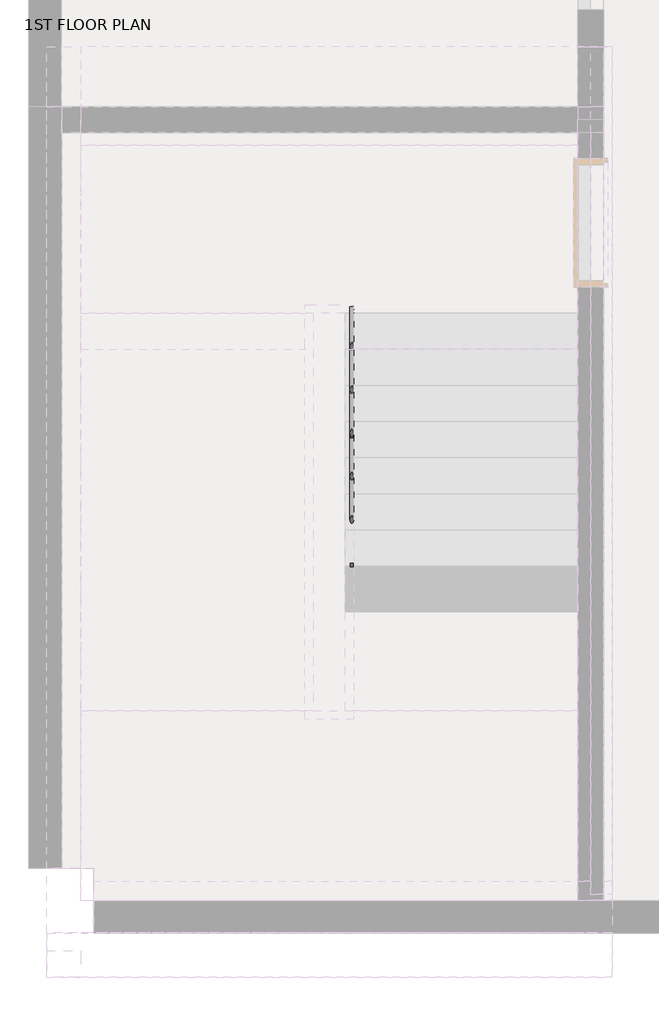
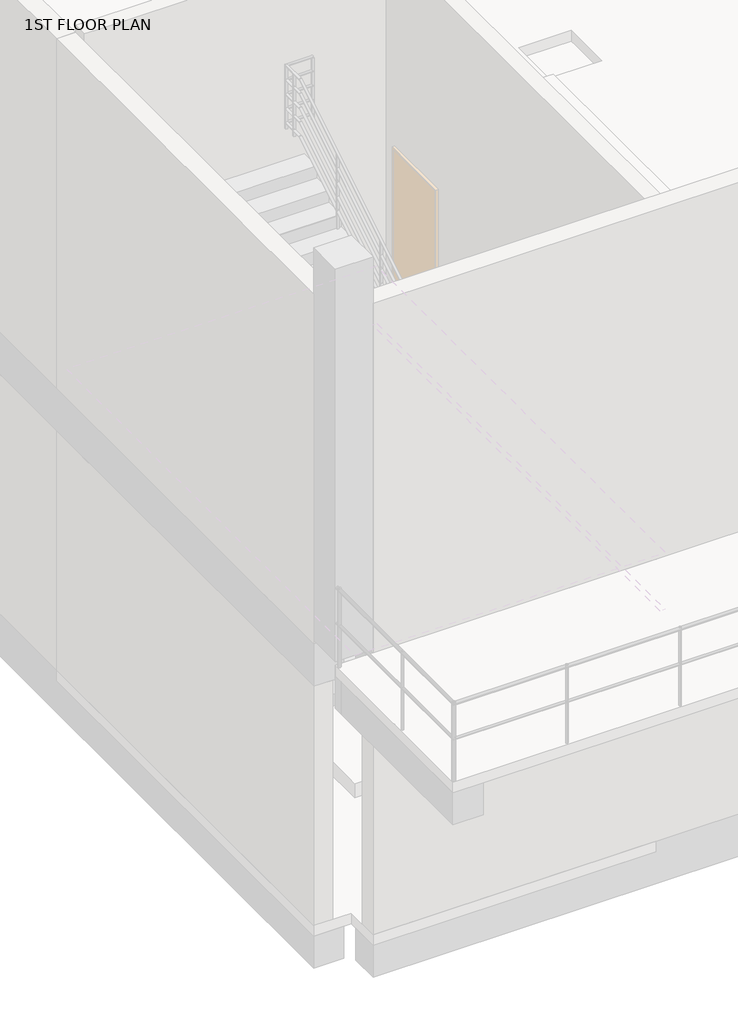
# One storey, part 7 of 9: 1 railing.
"""IFC4 building model written with IfcOpenShell, lengths in millimetres."""

from ifc_helpers import new_model, si_unit, frame, origin, place, context, project, spatial, polyline, circle_curve, ellipse_curve, outline, extrude, element, save
from ifc_brep_helpers import plane_surface, cylinder_surface, advanced_brep

model = new_model("IFC4")

# Units and contexts
model_context = context("Model", 3, world=origin())
ifc_project = project(units=[si_unit("LENGTHUNIT", "METRE", prefix="MILLI")], contexts=[model_context])

# Site, building, storey
site = spatial("IfcSite", under=ifc_project)
building = spatial("IfcBuilding", under=site)
storey = spatial("IfcBuildingStorey", under=building, Name="1ST FLOOR PLAN", Elevation=600.005241)

# Railing
placement = place(None, origin())
element("IfcRailing", 1, ObjectType="900mm 배관", at=placement, inside=storey, context=model_context, shape_type="SolidModel", body=[
    advanced_brep(
    [(2135.0, 25549.5208589, 1619.4537894), (2165.0, 25549.5208589, 1619.4537894), (2135.0, 22415.3944203, 3485.005241), (2165.0, 22415.3944203, 3485.005241), (2135.0, 22384.5208589, 3485.005241), (2165.0, 22354.5208589, 3485.005241), (1800.0, 22384.5208589, 3485.005241), (1800.0, 22354.5208589, 3485.005241)],
    [
        (0, 1, ellipse_curve(frame((2150.0, 25549.5208589, 1619.4537894), z_axis=(0.0, 1.0, 0.0), x_axis=(0.0, 0.0, -1.0)), 17.4562134, 15.0)),
        (1, 0, ellipse_curve(frame((2150.0, 25549.5208589, 1619.4537894), z_axis=(0.0, 1.0, 0.0), x_axis=(0.0, 0.0, -1.0)), 17.4562134, 15.0)),
        (0, 2),
        (2, 3, ellipse_curve(frame((2150.0, 22415.3944203, 3485.005241), z_axis=(0.0, 0.9641817474961643, -0.26524245096749255), x_axis=(0.0, -0.26524245096749166, -0.9641817474961646)), 15.5572329, 15.0)),
        (3, 1),
        (3, 2, ellipse_curve(frame((2150.0, 22415.3944203, 3485.005241), z_axis=(0.0, 0.9641817474961643, -0.26524245096749255), x_axis=(0.0, -0.26524245096749166, -0.9641817474961646)), 15.5572329, 15.0)),
        (2, 4),
        (4, 5, ellipse_curve(frame((2150.0, 22369.5208589, 3485.005241), z_axis=(0.7071067811865475, 0.7071067811865475, 0.0), x_axis=(-0.7071067811865474, 0.7071067811865476, 0.0)), 21.2132034, 15.0)),
        (5, 3),
        (5, 4, ellipse_curve(frame((2150.0, 22369.5208589, 3485.005241), z_axis=(0.7071067811865475, 0.7071067811865475, 0.0), x_axis=(-0.7071067811865474, 0.7071067811865476, 0.0)), 21.2132034, 15.0)),
        (6, 7, ellipse_curve(frame((1800.0, 22369.5208589, 3485.005241), z_axis=(-0.7071067811865476, 0.0, 0.7071067811865476), x_axis=(0.7071067811865474, 0.0, 0.7071067811865476)), 21.2132034, 15.0)),
        (7, 6, ellipse_curve(frame((1800.0, 22369.5208589, 3485.005241), z_axis=(-0.7071067811865476, 0.0, 0.7071067811865476), x_axis=(0.7071067811865474, 0.0, 0.7071067811865476)), 21.2132034, 15.0)),
        (4, 6),
        (7, 5),
    ],
    [
        plane_surface(frame((2150.0, 25549.5208589, 1636.9100029), z_axis=(0.0, 1.0, 0.0), x_axis=(0.0, 0.0, -1.0))),
        cylinder_surface(frame((2150.0, 25541.848601, 1624.0206096), z_axis=(0.0, 0.8592928844095147, -0.5114838597680054), x_axis=(1.0, 0.0, 0.0)), 15.0),
        cylinder_surface(frame((2150.0, 22419.5208589, 3485.005241), z_axis=(0.0, 1.0, 0.0), x_axis=(1.0, 0.0, 0.0)), 15.0),
        plane_surface(frame((1815.0, 22369.5208589, 3500.005241), z_axis=(-0.7071067811865476, 0.0, 0.7071067811865476), x_axis=(0.7071067811865476, 0.0, 0.7071067811865476))),
        cylinder_surface(frame((2150.0, 22369.5208589, 3485.005241), z_axis=(1.0, 0.0, 0.0), x_axis=(0.0, -1.0, 0.0)), 15.0),
    ],
    [
        (0, [[1, 2]]),
        (1, [[-1, 3, 4, 5]]),
        (1, [[-2, -5, 6, -3]]),
        (2, [[-4, 7, 8, 9]]),
        (2, [[-6, -9, 10, -7]]),
        (3, [[11, 12]]),
        (4, [[-8, 13, -12, 14]]),
        (4, [[-10, -14, -11, -13]]),
    ],
),
    advanced_brep(
    [(1800.0, 22384.5208589, 3485.005241), (1800.0, 22354.5208589, 3485.005241), (1800.0, 22384.5208589, 3610.9261474), (1800.0, 22354.5208589, 3627.9814314)],
    [
        (0, 1, ellipse_curve(frame((1800.0, 22369.5208589, 3485.005241), z_axis=(0.7071067811865476, 0.0, -0.7071067811865476), x_axis=(-0.7071067811865476, 0.0, -0.7071067811865474)), 21.2132034, 15.0)),
        (1, 0, ellipse_curve(frame((1800.0, 22369.5208589, 3485.005241), z_axis=(0.7071067811865476, 0.0, -0.7071067811865476), x_axis=(-0.7071067811865476, 0.0, -0.7071067811865474)), 21.2132034, 15.0)),
        (2, 3, ellipse_curve(frame((1800.0, 22369.5208589, 3619.4537894), z_axis=(0.0, 0.4942247162131791, 0.8693341876884877), x_axis=(0.0, 0.8693341876884879, -0.49422471621317876)), 17.2545843, 15.0)),
        (3, 2, ellipse_curve(frame((1800.0, 22369.5208589, 3619.4537894), z_axis=(0.0, 0.4942247162131791, 0.8693341876884877), x_axis=(0.0, 0.8693341876884879, -0.49422471621317876)), 17.2545843, 15.0)),
        (0, 2),
        (3, 1),
    ],
    [
        plane_surface(frame((1800.0, 22369.5208589, 3485.005241), z_axis=(0.7071067811865476, 0.0, -0.7071067811865476), x_axis=(0.7071067811865476, 0.0, 0.7071067811865476))),
        plane_surface(frame((1800.0, 22369.5208589, 3619.4537894), z_axis=(0.0, 0.4942247162131791, 0.8693341876884877), x_axis=(1.0, 0.0, 0.0))),
        cylinder_surface(frame((1800.0, 22369.5208589, 3485.005241), z_axis=(0.0, 0.0, -1.0), x_axis=(0.0, -1.0, 0.0)), 15.0),
    ],
    [
        (0, [[1, 2]]),
        (1, [[3, 4]]),
        (2, [[-1, 5, -4, 6]]),
        (2, [[-2, -6, -3, -5]]),
    ],
),
    advanced_brep(
    [(1815.0, 22369.5208589, 3619.4537894), (1785.0, 22369.5208589, 3619.4537894), (1815.0, 25503.6472975, 5485.005241), (1785.0, 25503.6472975, 5485.005241), (1815.0, 25534.5208589, 5485.005241), (1785.0, 25564.5208589, 5485.005241), (2150.0, 25534.5208589, 5485.005241), (2150.0, 25564.5208589, 5485.005241)],
    [
        (0, 1, ellipse_curve(frame((1800.0, 22369.5208589, 3619.4537894), z_axis=(0.0, -0.4942247162131791, -0.8693341876884877), x_axis=(0.0, -0.8693341876884876, 0.49422471621317926)), 17.2545843, 15.0)),
        (1, 0, ellipse_curve(frame((1800.0, 22369.5208589, 3619.4537894), z_axis=(0.0, -0.4942247162131791, -0.8693341876884877), x_axis=(0.0, -0.8693341876884876, 0.49422471621317926)), 17.2545843, 15.0)),
        (0, 2),
        (2, 3, ellipse_curve(frame((1800.0, 25503.6472975, 5485.005241), z_axis=(0.0, -0.9641817474961643, -0.26524245096749255), x_axis=(0.0, 0.26524245096749166, -0.9641817474961646)), 15.5572329, 15.0)),
        (3, 1),
        (3, 2, ellipse_curve(frame((1800.0, 25503.6472975, 5485.005241), z_axis=(0.0, -0.9641817474961643, -0.26524245096749255), x_axis=(0.0, 0.26524245096749166, -0.9641817474961646)), 15.5572329, 15.0)),
        (2, 4),
        (4, 5, ellipse_curve(frame((1800.0, 25549.5208589, 5485.005241), z_axis=(-0.7071067811865475, -0.7071067811865475, 0.0), x_axis=(0.7071067811865474, -0.7071067811865476, 0.0)), 21.2132034, 15.0)),
        (5, 3),
        (5, 4, ellipse_curve(frame((1800.0, 25549.5208589, 5485.005241), z_axis=(-0.7071067811865475, -0.7071067811865475, 0.0), x_axis=(0.7071067811865474, -0.7071067811865476, 0.0)), 21.2132034, 15.0)),
        (6, 7, circle_curve(frame((2150.0, 25549.5208589, 5485.005241), z_axis=(1.0, 0.0, 0.0), x_axis=(0.0, 1.0, 0.0)), 15.0)),
        (7, 6, circle_curve(frame((2150.0, 25549.5208589, 5485.005241), z_axis=(1.0, 0.0, 0.0), x_axis=(0.0, 1.0, 0.0)), 15.0)),
        (4, 6),
        (7, 5),
    ],
    [
        plane_surface(frame((1800.0, 22354.5208589, 3627.9814314), z_axis=(0.0, -0.4942247162131791, -0.8693341876884877), x_axis=(1.0, 0.0, 0.0))),
        cylinder_surface(frame((1800.0, 22362.1931168, 3615.0920382), z_axis=(0.0, -0.8592928844095147, -0.5114838597680054), x_axis=(-1.0, 0.0, 0.0)), 15.0),
        cylinder_surface(frame((1800.0, 25499.5208589, 5485.005241), z_axis=(0.0, -1.0, 0.0), x_axis=(-1.0, 0.0, 0.0)), 15.0),
        plane_surface(frame((2150.0, 25549.5208589, 5500.005241), z_axis=(1.0, 0.0, 0.0), x_axis=(0.0, 1.0, 0.0))),
        cylinder_surface(frame((1800.0, 25549.5208589, 5485.005241), z_axis=(-1.0, 0.0, 0.0), x_axis=(0.0, 1.0, 0.0)), 15.0),
    ],
    [
        (0, [[1, 2]]),
        (1, [[-1, 3, 4, 5]]),
        (1, [[-2, -5, 6, -3]]),
        (2, [[-4, 7, 8, 9]]),
        (2, [[-6, -9, 10, -7]]),
        (3, [[11, 12]]),
        (4, [[-8, 13, -12, 14]]),
        (4, [[-10, -14, -11, -13]]),
    ],
),
    advanced_brep(
    [(2165.0, 25549.5208589, 1419.4537894), (2135.0, 25549.5208589, 1419.4537894), (2165.0, 22415.3944203, 3285.005241), (2135.0, 22415.3944203, 3285.005241), (2165.0, 22384.5208589, 3285.005241), (2135.0, 22384.5208589, 3285.005241)],
    [
        (0, 1, ellipse_curve(frame((2150.0, 25549.5208589, 1419.4537894), z_axis=(0.0, 1.0, 0.0), x_axis=(0.0, 0.0, -1.0)), 17.4562134, 15.0)),
        (1, 0, ellipse_curve(frame((2150.0, 25549.5208589, 1419.4537894), z_axis=(0.0, 1.0, 0.0), x_axis=(0.0, 0.0, -1.0)), 17.4562134, 15.0)),
        (0, 2),
        (2, 3, ellipse_curve(frame((2150.0, 22415.3944203, 3285.005241), z_axis=(0.0, 0.9641817474961643, -0.26524245096749255), x_axis=(0.0, -0.26524245096749166, -0.9641817474961646)), 15.5572329, 15.0)),
        (3, 1),
        (3, 2, ellipse_curve(frame((2150.0, 22415.3944203, 3285.005241), z_axis=(0.0, 0.9641817474961643, -0.26524245096749255), x_axis=(0.0, -0.26524245096749166, -0.9641817474961646)), 15.5572329, 15.0)),
        (4, 5, circle_curve(frame((2150.0, 22384.5208589, 3285.005241), z_axis=(0.0, -1.0, 0.0), x_axis=(-1.0, 0.0, 0.0)), 15.0)),
        (5, 4, circle_curve(frame((2150.0, 22384.5208589, 3285.005241), z_axis=(0.0, -1.0, 0.0), x_axis=(-1.0, 0.0, 0.0)), 15.0)),
        (2, 4),
        (5, 3),
    ],
    [
        plane_surface(frame((2150.0, 25549.5208589, 1436.9100029), z_axis=(0.0, 1.0, 0.0), x_axis=(0.0, 0.0, -1.0))),
        cylinder_surface(frame((2150.0, 25541.848601, 1424.0206096), z_axis=(0.0, 0.8592928844095147, -0.5114838597680054), x_axis=(-1.0, 0.0, 0.0)), 15.0),
        plane_surface(frame((2150.0, 22384.5208589, 3300.005241), z_axis=(0.0, -1.0, 0.0), x_axis=(0.0, 0.0, -1.0))),
        cylinder_surface(frame((2150.0, 22419.5208589, 3285.005241), z_axis=(0.0, 1.0, 0.0), x_axis=(-1.0, 0.0, 0.0)), 15.0),
    ],
    [
        (0, [[1, 2]]),
        (1, [[-1, 3, 4, 5]]),
        (1, [[-2, -5, 6, -3]]),
        (2, [[7, 8]]),
        (3, [[-4, 9, -8, 10]]),
        (3, [[-6, -10, -7, -9]]),
    ],
),
    advanced_brep(
    [(2165.0, 22354.5208589, 3285.005241), (2165.0, 22384.5208589, 3285.005241), (1815.0, 22354.5208589, 3285.005241), (1815.0, 22384.5208589, 3285.005241)],
    [
        (0, 1, circle_curve(frame((2165.0, 22369.5208589, 3285.005241), z_axis=(1.0, 0.0, 0.0), x_axis=(0.0, 1.0, 0.0)), 15.0)),
        (1, 0, circle_curve(frame((2165.0, 22369.5208589, 3285.005241), z_axis=(1.0, 0.0, 0.0), x_axis=(0.0, 1.0, 0.0)), 15.0)),
        (2, 3, circle_curve(frame((1815.0, 22369.5208589, 3285.005241), z_axis=(-1.0, 0.0, 0.0), x_axis=(0.0, 1.0, 0.0)), 15.0)),
        (3, 2, circle_curve(frame((1815.0, 22369.5208589, 3285.005241), z_axis=(-1.0, 0.0, 0.0), x_axis=(0.0, 1.0, 0.0)), 15.0)),
        (0, 2),
        (3, 1),
    ],
    [
        plane_surface(frame((2165.0, 22369.5208589, 3300.005241), z_axis=(1.0, 0.0, 0.0), x_axis=(0.0, -1.0, 0.0))),
        plane_surface(frame((1815.0, 22369.5208589, 3300.005241), z_axis=(-1.0, 0.0, 0.0), x_axis=(0.0, -1.0, 0.0))),
        cylinder_surface(frame((2165.0, 22369.5208589, 3285.005241), z_axis=(1.0, 0.0, 0.0), x_axis=(0.0, 1.0, 0.0)), 15.0),
    ],
    [
        (0, [[1, 2]]),
        (1, [[3, 4]]),
        (2, [[-1, 5, -4, 6]]),
        (2, [[-2, -6, -3, -5]]),
    ],
),
    advanced_brep(
    [(1785.0, 22354.5208589, 3410.525218), (1815.0, 22354.5208589, 3410.525218), (1785.0, 25503.6472975, 5285.005241), (1815.0, 25503.6472975, 5285.005241), (1785.0, 25534.5208589, 5285.005241), (1815.0, 25534.5208589, 5285.005241)],
    [
        (0, 1, ellipse_curve(frame((1800.0, 22354.5208589, 3410.525218), z_axis=(0.0, -1.0, 0.0), x_axis=(0.0, 0.0, -1.0)), 17.4562134, 15.0)),
        (1, 0, ellipse_curve(frame((1800.0, 22354.5208589, 3410.525218), z_axis=(0.0, -1.0, 0.0), x_axis=(0.0, 0.0, -1.0)), 17.4562134, 15.0)),
        (0, 2),
        (2, 3, ellipse_curve(frame((1800.0, 25503.6472975, 5285.005241), z_axis=(0.0, -0.9641817474961643, -0.26524245096749255), x_axis=(0.0, 0.26524245096749166, -0.9641817474961646)), 15.5572329, 15.0)),
        (3, 1),
        (3, 2, ellipse_curve(frame((1800.0, 25503.6472975, 5285.005241), z_axis=(0.0, -0.9641817474961643, -0.26524245096749255), x_axis=(0.0, 0.26524245096749166, -0.9641817474961646)), 15.5572329, 15.0)),
        (4, 5, circle_curve(frame((1800.0, 25534.5208589, 5285.005241), z_axis=(0.0, 1.0, 0.0), x_axis=(1.0, 0.0, 0.0)), 15.0)),
        (5, 4, circle_curve(frame((1800.0, 25534.5208589, 5285.005241), z_axis=(0.0, 1.0, 0.0), x_axis=(1.0, 0.0, 0.0)), 15.0)),
        (2, 4),
        (5, 3),
    ],
    [
        plane_surface(frame((1800.0, 22354.5208589, 3427.9814314), z_axis=(0.0, -1.0, 0.0), x_axis=(0.0, 0.0, 1.0))),
        cylinder_surface(frame((1800.0, 22362.1931168, 3415.0920382), z_axis=(0.0, -0.8592928844095147, -0.5114838597680054), x_axis=(1.0, 0.0, 0.0)), 15.0),
        plane_surface(frame((1800.0, 25534.5208589, 5300.005241), z_axis=(0.0, 1.0, 0.0), x_axis=(0.0, 0.0, 1.0))),
        cylinder_surface(frame((1800.0, 25499.5208589, 5285.005241), z_axis=(0.0, -1.0, 0.0), x_axis=(1.0, 0.0, 0.0)), 15.0),
    ],
    [
        (0, [[1, 2]]),
        (1, [[-1, 3, 4, 5]]),
        (1, [[-2, -5, 6, -3]]),
        (2, [[7, 8]]),
        (3, [[-4, 9, -8, 10]]),
        (3, [[-6, -10, -7, -9]]),
    ],
),
    advanced_brep(
    [(1785.0, 25564.5208589, 5285.005241), (1785.0, 25534.5208589, 5285.005241), (2150.0, 25564.5208589, 5285.005241), (2150.0, 25534.5208589, 5285.005241)],
    [
        (0, 1, circle_curve(frame((1785.0, 25549.5208589, 5285.005241), z_axis=(-1.0, 0.0, 0.0), x_axis=(0.0, -1.0, 0.0)), 15.0)),
        (1, 0, circle_curve(frame((1785.0, 25549.5208589, 5285.005241), z_axis=(-1.0, 0.0, 0.0), x_axis=(0.0, -1.0, 0.0)), 15.0)),
        (2, 3, circle_curve(frame((2150.0, 25549.5208589, 5285.005241), z_axis=(1.0, 0.0, 0.0), x_axis=(0.0, -1.0, 0.0)), 15.0)),
        (3, 2, circle_curve(frame((2150.0, 25549.5208589, 5285.005241), z_axis=(1.0, 0.0, 0.0), x_axis=(0.0, -1.0, 0.0)), 15.0)),
        (0, 2),
        (3, 1),
    ],
    [
        plane_surface(frame((1785.0, 25549.5208589, 5300.005241), z_axis=(-1.0, 0.0, 0.0), x_axis=(0.0, 1.0, 0.0))),
        plane_surface(frame((2150.0, 25549.5208589, 5300.005241), z_axis=(1.0, 0.0, 0.0), x_axis=(0.0, 1.0, 0.0))),
        cylinder_surface(frame((1785.0, 25549.5208589, 5285.005241), z_axis=(-1.0, 0.0, 0.0), x_axis=(0.0, -1.0, 0.0)), 15.0),
    ],
    [
        (0, [[1, 2]]),
        (1, [[3, 4]]),
        (2, [[-1, 5, -4, 6]]),
        (2, [[-2, -6, -3, -5]]),
    ],
),
    advanced_brep(
    [(2165.0, 25549.5208589, 1219.4537894), (2135.0, 25549.5208589, 1219.4537894), (2165.0, 22415.3944203, 3085.005241), (2135.0, 22415.3944203, 3085.005241), (2165.0, 22384.5208589, 3085.005241), (2135.0, 22384.5208589, 3085.005241)],
    [
        (0, 1, ellipse_curve(frame((2150.0, 25549.5208589, 1219.4537894), z_axis=(0.0, 1.0, 0.0), x_axis=(0.0, 0.0, -1.0)), 17.4562134, 15.0)),
        (1, 0, ellipse_curve(frame((2150.0, 25549.5208589, 1219.4537894), z_axis=(0.0, 1.0, 0.0), x_axis=(0.0, 0.0, -1.0)), 17.4562134, 15.0)),
        (0, 2),
        (2, 3, ellipse_curve(frame((2150.0, 22415.3944203, 3085.005241), z_axis=(0.0, 0.9641817474961643, -0.26524245096749255), x_axis=(0.0, -0.26524245096749166, -0.9641817474961646)), 15.5572329, 15.0)),
        (3, 1),
        (3, 2, ellipse_curve(frame((2150.0, 22415.3944203, 3085.005241), z_axis=(0.0, 0.9641817474961643, -0.26524245096749255), x_axis=(0.0, -0.26524245096749166, -0.9641817474961646)), 15.5572329, 15.0)),
        (4, 5, circle_curve(frame((2150.0, 22384.5208589, 3085.005241), z_axis=(0.0, -1.0, 0.0), x_axis=(-1.0, 0.0, 0.0)), 15.0)),
        (5, 4, circle_curve(frame((2150.0, 22384.5208589, 3085.005241), z_axis=(0.0, -1.0, 0.0), x_axis=(-1.0, 0.0, 0.0)), 15.0)),
        (2, 4),
        (5, 3),
    ],
    [
        plane_surface(frame((2150.0, 25549.5208589, 1236.9100029), z_axis=(0.0, 1.0, 0.0), x_axis=(0.0, 0.0, -1.0))),
        cylinder_surface(frame((2150.0, 25541.848601, 1224.0206096), z_axis=(0.0, 0.8592928844095147, -0.5114838597680054), x_axis=(-1.0, 0.0, 0.0)), 15.0),
        plane_surface(frame((2150.0, 22384.5208589, 3100.005241), z_axis=(0.0, -1.0, 0.0), x_axis=(0.0, 0.0, -1.0))),
        cylinder_surface(frame((2150.0, 22419.5208589, 3085.005241), z_axis=(0.0, 1.0, 0.0), x_axis=(-1.0, 0.0, 0.0)), 15.0),
    ],
    [
        (0, [[1, 2]]),
        (1, [[-1, 3, 4, 5]]),
        (1, [[-2, -5, 6, -3]]),
        (2, [[7, 8]]),
        (3, [[-4, 9, -8, 10]]),
        (3, [[-6, -10, -7, -9]]),
    ],
),
    advanced_brep(
    [(2165.0, 22354.5208589, 3085.005241), (2165.0, 22384.5208589, 3085.005241), (1815.0, 22354.5208589, 3085.005241), (1815.0, 22384.5208589, 3085.005241)],
    [
        (0, 1, circle_curve(frame((2165.0, 22369.5208589, 3085.005241), z_axis=(1.0, 0.0, 0.0), x_axis=(0.0, 1.0, 0.0)), 15.0)),
        (1, 0, circle_curve(frame((2165.0, 22369.5208589, 3085.005241), z_axis=(1.0, 0.0, 0.0), x_axis=(0.0, 1.0, 0.0)), 15.0)),
        (2, 3, circle_curve(frame((1815.0, 22369.5208589, 3085.005241), z_axis=(-1.0, 0.0, 0.0), x_axis=(0.0, 1.0, 0.0)), 15.0)),
        (3, 2, circle_curve(frame((1815.0, 22369.5208589, 3085.005241), z_axis=(-1.0, 0.0, 0.0), x_axis=(0.0, 1.0, 0.0)), 15.0)),
        (0, 2),
        (3, 1),
    ],
    [
        plane_surface(frame((2165.0, 22369.5208589, 3100.005241), z_axis=(1.0, 0.0, 0.0), x_axis=(0.0, -1.0, 0.0))),
        plane_surface(frame((1815.0, 22369.5208589, 3100.005241), z_axis=(-1.0, 0.0, 0.0), x_axis=(0.0, -1.0, 0.0))),
        cylinder_surface(frame((2165.0, 22369.5208589, 3085.005241), z_axis=(1.0, 0.0, 0.0), x_axis=(0.0, 1.0, 0.0)), 15.0),
    ],
    [
        (0, [[1, 2]]),
        (1, [[3, 4]]),
        (2, [[-1, 5, -4, 6]]),
        (2, [[-2, -6, -3, -5]]),
    ],
),
    advanced_brep(
    [(1785.0, 22354.5208589, 3210.525218), (1815.0, 22354.5208589, 3210.525218), (1785.0, 25503.6472975, 5085.005241), (1815.0, 25503.6472975, 5085.005241), (1785.0, 25534.5208589, 5085.005241), (1815.0, 25534.5208589, 5085.005241)],
    [
        (0, 1, ellipse_curve(frame((1800.0, 22354.5208589, 3210.525218), z_axis=(0.0, -1.0, 0.0), x_axis=(0.0, 0.0, -1.0)), 17.4562134, 15.0)),
        (1, 0, ellipse_curve(frame((1800.0, 22354.5208589, 3210.525218), z_axis=(0.0, -1.0, 0.0), x_axis=(0.0, 0.0, -1.0)), 17.4562134, 15.0)),
        (0, 2),
        (2, 3, ellipse_curve(frame((1800.0, 25503.6472975, 5085.005241), z_axis=(0.0, -0.9641817474961643, -0.26524245096749255), x_axis=(0.0, 0.26524245096749166, -0.9641817474961646)), 15.5572329, 15.0)),
        (3, 1),
        (3, 2, ellipse_curve(frame((1800.0, 25503.6472975, 5085.005241), z_axis=(0.0, -0.9641817474961643, -0.26524245096749255), x_axis=(0.0, 0.26524245096749166, -0.9641817474961646)), 15.5572329, 15.0)),
        (4, 5, circle_curve(frame((1800.0, 25534.5208589, 5085.005241), z_axis=(0.0, 1.0, 0.0), x_axis=(1.0, 0.0, 0.0)), 15.0)),
        (5, 4, circle_curve(frame((1800.0, 25534.5208589, 5085.005241), z_axis=(0.0, 1.0, 0.0), x_axis=(1.0, 0.0, 0.0)), 15.0)),
        (2, 4),
        (5, 3),
    ],
    [
        plane_surface(frame((1800.0, 22354.5208589, 3227.9814314), z_axis=(0.0, -1.0, 0.0), x_axis=(0.0, 0.0, 1.0))),
        cylinder_surface(frame((1800.0, 22362.1931168, 3215.0920382), z_axis=(0.0, -0.8592928844095147, -0.5114838597680054), x_axis=(1.0, 0.0, 0.0)), 15.0),
        plane_surface(frame((1800.0, 25534.5208589, 5100.005241), z_axis=(0.0, 1.0, 0.0), x_axis=(0.0, 0.0, 1.0))),
        cylinder_surface(frame((1800.0, 25499.5208589, 5085.005241), z_axis=(0.0, -1.0, 0.0), x_axis=(1.0, 0.0, 0.0)), 15.0),
    ],
    [
        (0, [[1, 2]]),
        (1, [[-1, 3, 4, 5]]),
        (1, [[-2, -5, 6, -3]]),
        (2, [[7, 8]]),
        (3, [[-4, 9, -8, 10]]),
        (3, [[-6, -10, -7, -9]]),
    ],
),
    advanced_brep(
    [(1785.0, 25564.5208589, 5085.005241), (1785.0, 25534.5208589, 5085.005241), (2150.0, 25564.5208589, 5085.005241), (2150.0, 25534.5208589, 5085.005241)],
    [
        (0, 1, circle_curve(frame((1785.0, 25549.5208589, 5085.005241), z_axis=(-1.0, 0.0, 0.0), x_axis=(0.0, -1.0, 0.0)), 15.0)),
        (1, 0, circle_curve(frame((1785.0, 25549.5208589, 5085.005241), z_axis=(-1.0, 0.0, 0.0), x_axis=(0.0, -1.0, 0.0)), 15.0)),
        (2, 3, circle_curve(frame((2150.0, 25549.5208589, 5085.005241), z_axis=(1.0, 0.0, 0.0), x_axis=(0.0, -1.0, 0.0)), 15.0)),
        (3, 2, circle_curve(frame((2150.0, 25549.5208589, 5085.005241), z_axis=(1.0, 0.0, 0.0), x_axis=(0.0, -1.0, 0.0)), 15.0)),
        (0, 2),
        (3, 1),
    ],
    [
        plane_surface(frame((1785.0, 25549.5208589, 5100.005241), z_axis=(-1.0, 0.0, 0.0), x_axis=(0.0, 1.0, 0.0))),
        plane_surface(frame((2150.0, 25549.5208589, 5100.005241), z_axis=(1.0, 0.0, 0.0), x_axis=(0.0, 1.0, 0.0))),
        cylinder_surface(frame((1785.0, 25549.5208589, 5085.005241), z_axis=(-1.0, 0.0, 0.0), x_axis=(0.0, -1.0, 0.0)), 15.0),
    ],
    [
        (0, [[1, 2]]),
        (1, [[3, 4]]),
        (2, [[-1, 5, -4, 6]]),
        (2, [[-2, -6, -3, -5]]),
    ],
),
    advanced_brep(
    [(2165.0, 25549.5208589, 1019.4537894), (2135.0, 25549.5208589, 1019.4537894), (2165.0, 22415.3944203, 2885.005241), (2135.0, 22415.3944203, 2885.005241), (2165.0, 22384.5208589, 2885.005241), (2135.0, 22384.5208589, 2885.005241)],
    [
        (0, 1, ellipse_curve(frame((2150.0, 25549.5208589, 1019.4537894), z_axis=(0.0, 1.0, 0.0), x_axis=(0.0, 0.0, -1.0)), 17.4562134, 15.0)),
        (1, 0, ellipse_curve(frame((2150.0, 25549.5208589, 1019.4537894), z_axis=(0.0, 1.0, 0.0), x_axis=(0.0, 0.0, -1.0)), 17.4562134, 15.0)),
        (0, 2),
        (2, 3, ellipse_curve(frame((2150.0, 22415.3944203, 2885.005241), z_axis=(0.0, 0.9641817474961643, -0.26524245096749255), x_axis=(0.0, -0.26524245096749166, -0.9641817474961646)), 15.5572329, 15.0)),
        (3, 1),
        (3, 2, ellipse_curve(frame((2150.0, 22415.3944203, 2885.005241), z_axis=(0.0, 0.9641817474961643, -0.26524245096749255), x_axis=(0.0, -0.26524245096749166, -0.9641817474961646)), 15.5572329, 15.0)),
        (4, 5, circle_curve(frame((2150.0, 22384.5208589, 2885.005241), z_axis=(0.0, -1.0, 0.0), x_axis=(-1.0, 0.0, 0.0)), 15.0)),
        (5, 4, circle_curve(frame((2150.0, 22384.5208589, 2885.005241), z_axis=(0.0, -1.0, 0.0), x_axis=(-1.0, 0.0, 0.0)), 15.0)),
        (2, 4),
        (5, 3),
    ],
    [
        plane_surface(frame((2150.0, 25549.5208589, 1036.9100029), z_axis=(0.0, 1.0, 0.0), x_axis=(0.0, 0.0, -1.0))),
        cylinder_surface(frame((2150.0, 25541.848601, 1024.0206096), z_axis=(0.0, 0.8592928844095147, -0.5114838597680054), x_axis=(-1.0, 0.0, 0.0)), 15.0),
        plane_surface(frame((2150.0, 22384.5208589, 2900.005241), z_axis=(0.0, -1.0, 0.0), x_axis=(0.0, 0.0, -1.0))),
        cylinder_surface(frame((2150.0, 22419.5208589, 2885.005241), z_axis=(0.0, 1.0, 0.0), x_axis=(-1.0, 0.0, 0.0)), 15.0),
    ],
    [
        (0, [[1, 2]]),
        (1, [[-1, 3, 4, 5]]),
        (1, [[-2, -5, 6, -3]]),
        (2, [[7, 8]]),
        (3, [[-4, 9, -8, 10]]),
        (3, [[-6, -10, -7, -9]]),
    ],
),
    advanced_brep(
    [(2165.0, 22354.5208589, 2885.005241), (2165.0, 22384.5208589, 2885.005241), (1815.0, 22354.5208589, 2885.005241), (1815.0, 22384.5208589, 2885.005241)],
    [
        (0, 1, circle_curve(frame((2165.0, 22369.5208589, 2885.005241), z_axis=(1.0, 0.0, 0.0), x_axis=(0.0, 1.0, 0.0)), 15.0)),
        (1, 0, circle_curve(frame((2165.0, 22369.5208589, 2885.005241), z_axis=(1.0, 0.0, 0.0), x_axis=(0.0, 1.0, 0.0)), 15.0)),
        (2, 3, circle_curve(frame((1815.0, 22369.5208589, 2885.005241), z_axis=(-1.0, 0.0, 0.0), x_axis=(0.0, 1.0, 0.0)), 15.0)),
        (3, 2, circle_curve(frame((1815.0, 22369.5208589, 2885.005241), z_axis=(-1.0, 0.0, 0.0), x_axis=(0.0, 1.0, 0.0)), 15.0)),
        (0, 2),
        (3, 1),
    ],
    [
        plane_surface(frame((2165.0, 22369.5208589, 2900.005241), z_axis=(1.0, 0.0, 0.0), x_axis=(0.0, -1.0, 0.0))),
        plane_surface(frame((1815.0, 22369.5208589, 2900.005241), z_axis=(-1.0, 0.0, 0.0), x_axis=(0.0, -1.0, 0.0))),
        cylinder_surface(frame((2165.0, 22369.5208589, 2885.005241), z_axis=(1.0, 0.0, 0.0), x_axis=(0.0, 1.0, 0.0)), 15.0),
    ],
    [
        (0, [[1, 2]]),
        (1, [[3, 4]]),
        (2, [[-1, 5, -4, 6]]),
        (2, [[-2, -6, -3, -5]]),
    ],
),
    advanced_brep(
    [(1785.0, 22354.5208589, 3010.525218), (1815.0, 22354.5208589, 3010.525218), (1785.0, 25503.6472975, 4885.005241), (1815.0, 25503.6472975, 4885.005241), (1785.0, 25534.5208589, 4885.005241), (1815.0, 25534.5208589, 4885.005241)],
    [
        (0, 1, ellipse_curve(frame((1800.0, 22354.5208589, 3010.525218), z_axis=(0.0, -1.0, 0.0), x_axis=(0.0, 0.0, -1.0)), 17.4562134, 15.0)),
        (1, 0, ellipse_curve(frame((1800.0, 22354.5208589, 3010.525218), z_axis=(0.0, -1.0, 0.0), x_axis=(0.0, 0.0, -1.0)), 17.4562134, 15.0)),
        (0, 2),
        (2, 3, ellipse_curve(frame((1800.0, 25503.6472975, 4885.005241), z_axis=(0.0, -0.9641817474961643, -0.26524245096749255), x_axis=(0.0, 0.26524245096749166, -0.9641817474961646)), 15.5572329, 15.0)),
        (3, 1),
        (3, 2, ellipse_curve(frame((1800.0, 25503.6472975, 4885.005241), z_axis=(0.0, -0.9641817474961643, -0.26524245096749255), x_axis=(0.0, 0.26524245096749166, -0.9641817474961646)), 15.5572329, 15.0)),
        (4, 5, circle_curve(frame((1800.0, 25534.5208589, 4885.005241), z_axis=(0.0, 1.0, 0.0), x_axis=(1.0, 0.0, 0.0)), 15.0)),
        (5, 4, circle_curve(frame((1800.0, 25534.5208589, 4885.005241), z_axis=(0.0, 1.0, 0.0), x_axis=(1.0, 0.0, 0.0)), 15.0)),
        (2, 4),
        (5, 3),
    ],
    [
        plane_surface(frame((1800.0, 22354.5208589, 3027.9814314), z_axis=(0.0, -1.0, 0.0), x_axis=(0.0, 0.0, 1.0))),
        cylinder_surface(frame((1800.0, 22362.1931168, 3015.0920382), z_axis=(0.0, -0.8592928844095147, -0.5114838597680054), x_axis=(1.0, 0.0, 0.0)), 15.0),
        plane_surface(frame((1800.0, 25534.5208589, 4900.005241), z_axis=(0.0, 1.0, 0.0), x_axis=(0.0, 0.0, 1.0))),
        cylinder_surface(frame((1800.0, 25499.5208589, 4885.005241), z_axis=(0.0, -1.0, 0.0), x_axis=(1.0, 0.0, 0.0)), 15.0),
    ],
    [
        (0, [[1, 2]]),
        (1, [[-1, 3, 4, 5]]),
        (1, [[-2, -5, 6, -3]]),
        (2, [[7, 8]]),
        (3, [[-4, 9, -8, 10]]),
        (3, [[-6, -10, -7, -9]]),
    ],
),
    advanced_brep(
    [(1785.0, 25564.5208589, 4885.005241), (1785.0, 25534.5208589, 4885.005241), (2150.0, 25564.5208589, 4885.005241), (2150.0, 25534.5208589, 4885.005241)],
    [
        (0, 1, circle_curve(frame((1785.0, 25549.5208589, 4885.005241), z_axis=(-1.0, 0.0, 0.0), x_axis=(0.0, -1.0, 0.0)), 15.0)),
        (1, 0, circle_curve(frame((1785.0, 25549.5208589, 4885.005241), z_axis=(-1.0, 0.0, 0.0), x_axis=(0.0, -1.0, 0.0)), 15.0)),
        (2, 3, circle_curve(frame((2150.0, 25549.5208589, 4885.005241), z_axis=(1.0, 0.0, 0.0), x_axis=(0.0, -1.0, 0.0)), 15.0)),
        (3, 2, circle_curve(frame((2150.0, 25549.5208589, 4885.005241), z_axis=(1.0, 0.0, 0.0), x_axis=(0.0, -1.0, 0.0)), 15.0)),
        (0, 2),
        (3, 1),
    ],
    [
        plane_surface(frame((1785.0, 25549.5208589, 4900.005241), z_axis=(-1.0, 0.0, 0.0), x_axis=(0.0, 1.0, 0.0))),
        plane_surface(frame((2150.0, 25549.5208589, 4900.005241), z_axis=(1.0, 0.0, 0.0), x_axis=(0.0, 1.0, 0.0))),
        cylinder_surface(frame((1785.0, 25549.5208589, 4885.005241), z_axis=(-1.0, 0.0, 0.0), x_axis=(0.0, -1.0, 0.0)), 15.0),
    ],
    [
        (0, [[1, 2]]),
        (1, [[3, 4]]),
        (2, [[-1, 5, -4, 6]]),
        (2, [[-2, -6, -3, -5]]),
    ],
),
    advanced_brep(
    [(2165.0, 25549.5208589, 819.4537894), (2135.0, 25549.5208589, 819.4537894), (2165.0, 22415.3944203, 2685.005241), (2135.0, 22415.3944203, 2685.005241), (2165.0, 22384.5208589, 2685.005241), (2135.0, 22384.5208589, 2685.005241)],
    [
        (0, 1, ellipse_curve(frame((2150.0, 25549.5208589, 819.4537894), z_axis=(0.0, 1.0, 0.0), x_axis=(0.0, 0.0, -1.0)), 17.4562134, 15.0)),
        (1, 0, ellipse_curve(frame((2150.0, 25549.5208589, 819.4537894), z_axis=(0.0, 1.0, 0.0), x_axis=(0.0, 0.0, -1.0)), 17.4562134, 15.0)),
        (0, 2),
        (2, 3, ellipse_curve(frame((2150.0, 22415.3944203, 2685.005241), z_axis=(0.0, 0.9641817474961643, -0.26524245096749255), x_axis=(0.0, -0.26524245096749166, -0.9641817474961646)), 15.5572329, 15.0)),
        (3, 1),
        (3, 2, ellipse_curve(frame((2150.0, 22415.3944203, 2685.005241), z_axis=(0.0, 0.9641817474961643, -0.26524245096749255), x_axis=(0.0, -0.26524245096749166, -0.9641817474961646)), 15.5572329, 15.0)),
        (4, 5, circle_curve(frame((2150.0, 22384.5208589, 2685.005241), z_axis=(0.0, -1.0, 0.0), x_axis=(-1.0, 0.0, 0.0)), 15.0)),
        (5, 4, circle_curve(frame((2150.0, 22384.5208589, 2685.005241), z_axis=(0.0, -1.0, 0.0), x_axis=(-1.0, 0.0, 0.0)), 15.0)),
        (2, 4),
        (5, 3),
    ],
    [
        plane_surface(frame((2150.0, 25549.5208589, 836.9100029), z_axis=(0.0, 1.0, 0.0), x_axis=(0.0, 0.0, -1.0))),
        cylinder_surface(frame((2150.0, 25541.848601, 824.0206096), z_axis=(0.0, 0.8592928844095147, -0.5114838597680054), x_axis=(-1.0, 0.0, 0.0)), 15.0),
        plane_surface(frame((2150.0, 22384.5208589, 2700.005241), z_axis=(0.0, -1.0, 0.0), x_axis=(0.0, 0.0, -1.0))),
        cylinder_surface(frame((2150.0, 22419.5208589, 2685.005241), z_axis=(0.0, 1.0, 0.0), x_axis=(-1.0, 0.0, 0.0)), 15.0),
    ],
    [
        (0, [[1, 2]]),
        (1, [[-1, 3, 4, 5]]),
        (1, [[-2, -5, 6, -3]]),
        (2, [[7, 8]]),
        (3, [[-4, 9, -8, 10]]),
        (3, [[-6, -10, -7, -9]]),
    ],
),
    advanced_brep(
    [(2165.0, 22354.5208589, 2685.005241), (2165.0, 22384.5208589, 2685.005241), (1815.0, 22354.5208589, 2685.005241), (1815.0, 22384.5208589, 2685.005241)],
    [
        (0, 1, circle_curve(frame((2165.0, 22369.5208589, 2685.005241), z_axis=(1.0, 0.0, 0.0), x_axis=(0.0, 1.0, 0.0)), 15.0)),
        (1, 0, circle_curve(frame((2165.0, 22369.5208589, 2685.005241), z_axis=(1.0, 0.0, 0.0), x_axis=(0.0, 1.0, 0.0)), 15.0)),
        (2, 3, circle_curve(frame((1815.0, 22369.5208589, 2685.005241), z_axis=(-1.0, 0.0, 0.0), x_axis=(0.0, 1.0, 0.0)), 15.0)),
        (3, 2, circle_curve(frame((1815.0, 22369.5208589, 2685.005241), z_axis=(-1.0, 0.0, 0.0), x_axis=(0.0, 1.0, 0.0)), 15.0)),
        (0, 2),
        (3, 1),
    ],
    [
        plane_surface(frame((2165.0, 22369.5208589, 2700.005241), z_axis=(1.0, 0.0, 0.0), x_axis=(0.0, -1.0, 0.0))),
        plane_surface(frame((1815.0, 22369.5208589, 2700.005241), z_axis=(-1.0, 0.0, 0.0), x_axis=(0.0, -1.0, 0.0))),
        cylinder_surface(frame((2165.0, 22369.5208589, 2685.005241), z_axis=(1.0, 0.0, 0.0), x_axis=(0.0, 1.0, 0.0)), 15.0),
    ],
    [
        (0, [[1, 2]]),
        (1, [[3, 4]]),
        (2, [[-1, 5, -4, 6]]),
        (2, [[-2, -6, -3, -5]]),
    ],
),
    advanced_brep(
    [(1785.0, 22354.5208589, 2810.525218), (1815.0, 22354.5208589, 2810.525218), (1785.0, 25503.6472975, 4685.005241), (1815.0, 25503.6472975, 4685.005241), (1785.0, 25534.5208589, 4685.005241), (1815.0, 25534.5208589, 4685.005241)],
    [
        (0, 1, ellipse_curve(frame((1800.0, 22354.5208589, 2810.525218), z_axis=(0.0, -1.0, 0.0), x_axis=(0.0, 0.0, -1.0)), 17.4562134, 15.0)),
        (1, 0, ellipse_curve(frame((1800.0, 22354.5208589, 2810.525218), z_axis=(0.0, -1.0, 0.0), x_axis=(0.0, 0.0, -1.0)), 17.4562134, 15.0)),
        (0, 2),
        (2, 3, ellipse_curve(frame((1800.0, 25503.6472975, 4685.005241), z_axis=(0.0, -0.9641817474961643, -0.26524245096749255), x_axis=(0.0, 0.26524245096749166, -0.9641817474961646)), 15.5572329, 15.0)),
        (3, 1),
        (3, 2, ellipse_curve(frame((1800.0, 25503.6472975, 4685.005241), z_axis=(0.0, -0.9641817474961643, -0.26524245096749255), x_axis=(0.0, 0.26524245096749166, -0.9641817474961646)), 15.5572329, 15.0)),
        (4, 5, circle_curve(frame((1800.0, 25534.5208589, 4685.005241), z_axis=(0.0, 1.0, 0.0), x_axis=(1.0, 0.0, 0.0)), 15.0)),
        (5, 4, circle_curve(frame((1800.0, 25534.5208589, 4685.005241), z_axis=(0.0, 1.0, 0.0), x_axis=(1.0, 0.0, 0.0)), 15.0)),
        (2, 4),
        (5, 3),
    ],
    [
        plane_surface(frame((1800.0, 22354.5208589, 2827.9814314), z_axis=(0.0, -1.0, 0.0), x_axis=(0.0, 0.0, 1.0))),
        cylinder_surface(frame((1800.0, 22362.1931168, 2815.0920382), z_axis=(0.0, -0.8592928844095147, -0.5114838597680054), x_axis=(1.0, 0.0, 0.0)), 15.0),
        plane_surface(frame((1800.0, 25534.5208589, 4700.005241), z_axis=(0.0, 1.0, 0.0), x_axis=(0.0, 0.0, 1.0))),
        cylinder_surface(frame((1800.0, 25499.5208589, 4685.005241), z_axis=(0.0, -1.0, 0.0), x_axis=(1.0, 0.0, 0.0)), 15.0),
    ],
    [
        (0, [[1, 2]]),
        (1, [[-1, 3, 4, 5]]),
        (1, [[-2, -5, 6, -3]]),
        (2, [[7, 8]]),
        (3, [[-4, 9, -8, 10]]),
        (3, [[-6, -10, -7, -9]]),
    ],
),
    advanced_brep(
    [(1785.0, 25564.5208589, 4685.005241), (1785.0, 25534.5208589, 4685.005241), (2150.0, 25564.5208589, 4685.005241), (2150.0, 25534.5208589, 4685.005241)],
    [
        (0, 1, circle_curve(frame((1785.0, 25549.5208589, 4685.005241), z_axis=(-1.0, 0.0, 0.0), x_axis=(0.0, -1.0, 0.0)), 15.0)),
        (1, 0, circle_curve(frame((1785.0, 25549.5208589, 4685.005241), z_axis=(-1.0, 0.0, 0.0), x_axis=(0.0, -1.0, 0.0)), 15.0)),
        (2, 3, circle_curve(frame((2150.0, 25549.5208589, 4685.005241), z_axis=(1.0, 0.0, 0.0), x_axis=(0.0, -1.0, 0.0)), 15.0)),
        (3, 2, circle_curve(frame((2150.0, 25549.5208589, 4685.005241), z_axis=(1.0, 0.0, 0.0), x_axis=(0.0, -1.0, 0.0)), 15.0)),
        (0, 2),
        (3, 1),
    ],
    [
        plane_surface(frame((1785.0, 25549.5208589, 4700.005241), z_axis=(-1.0, 0.0, 0.0), x_axis=(0.0, 1.0, 0.0))),
        plane_surface(frame((2150.0, 25549.5208589, 4700.005241), z_axis=(1.0, 0.0, 0.0), x_axis=(0.0, 1.0, 0.0))),
        cylinder_surface(frame((1785.0, 25549.5208589, 4685.005241), z_axis=(-1.0, 0.0, 0.0), x_axis=(0.0, -1.0, 0.0)), 15.0),
    ],
    [
        (0, [[1, 2]]),
        (1, [[3, 4]]),
        (2, [[-1, 5, -4, 6]]),
        (2, [[-2, -6, -3, -5]]),
    ],
),
    extrude(outline(polyline([(25357.0208589, 5380.2713855), (25382.0208589, 5395.1523379), (25382.0208589, 4433.3385743), (25357.0208589, 4433.3385743), (25357.0208589, 5380.2713855)])), frame((1787.5, 0.0, 0.0), z_axis=(1.0, 0.0, 0.0), x_axis=(0.0, 1.0, 0.0)), (0.0, 0.0, 1.0), 25.0),
    extrude(outline(polyline([(24357.0208589, 4785.0332903), (24382.0208589, 4799.9142427), (24382.0208589, 3766.6719076), (24357.0208589, 3766.6719076), (24357.0208589, 4785.0332903)])), frame((1787.5, 0.0, 0.0), z_axis=(1.0, 0.0, 0.0), x_axis=(0.0, 1.0, 0.0)), (0.0, 0.0, 1.0), 25.0),
    extrude(outline(polyline([(23357.0208589, 4189.795195), (23382.0208589, 4204.6761474), (23382.0208589, 3266.6719076), (23357.0208589, 3266.6719076), (23357.0208589, 4189.795195)])), frame((1787.5, 0.0, 0.0), z_axis=(1.0, 0.0, 0.0), x_axis=(0.0, 1.0, 0.0)), (0.0, 0.0, 1.0), 25.0),
    extrude(outline(polyline([(22537.0208589, 3395.1523379), (22562.0208589, 3380.2713855), (22562.0208589, 2433.3385743), (22537.0208589, 2433.3385743), (22537.0208589, 3395.1523379)])), frame((2137.5, 0.0, 0.0), z_axis=(1.0, 0.0, 0.0), x_axis=(0.0, 1.0, 0.0)), (0.0, 0.0, 1.0), 25.0),
    extrude(outline(polyline([(23537.0208589, 2799.9142427), (23562.0208589, 2785.0332903), (23562.0208589, 1766.6719076), (23537.0208589, 1766.6719076), (23537.0208589, 2799.9142427)])), frame((2137.5, 0.0, 0.0), z_axis=(1.0, 0.0, 0.0), x_axis=(0.0, 1.0, 0.0)), (0.0, 0.0, 1.0), 25.0),
    extrude(outline(polyline([(24537.0208589, 2204.6761474), (24562.0208589, 2189.795195), (24562.0208589, 1266.6719076), (24537.0208589, 1266.6719076), (24537.0208589, 2204.6761474)])), frame((2137.5, 0.0, 0.0), z_axis=(1.0, 0.0, 0.0), x_axis=(0.0, 1.0, 0.0)), (0.0, 0.0, 1.0), 25.0),
    extrude(outline(polyline([(2137.5, 25537.0208589), (2137.5, 25562.0208589), (2162.5, 25562.0208589), (2162.5, 25537.0208589), (2137.5, 25537.0208589)])), frame((0.0, 0.0, 4600.005241), z_axis=(0.0, 0.0, 1.0), x_axis=(1.0, 0.0, 0.0)), (0.0, 0.0, 1.0), 870.0),
    extrude(outline(polyline([(1812.5, 25537.0208589), (1787.5, 25537.0208589), (1787.5, 25562.0208589), (1812.5, 25562.0208589), (1812.5, 25537.0208589)])), frame((0.0, 0.0, 4600.005241), z_axis=(0.0, 0.0, 1.0), x_axis=(1.0, 0.0, 0.0)), (0.0, 0.0, 1.0), 870.0),
    extrude(outline(polyline([(1812.5, 22382.0208589), (1812.5, 22357.0208589), (1787.5, 22357.0208589), (1787.5, 22382.0208589), (1812.5, 22382.0208589)])), frame((0.0, 0.0, 2600.005241), z_axis=(0.0, 0.0, 1.0), x_axis=(1.0, 0.0, 0.0)), (0.0, 0.0, 1.0), 870.0),
    extrude(outline(polyline([(2137.5, 22382.0208589), (2162.5, 22382.0208589), (2162.5, 22357.0208589), (2137.5, 22357.0208589), (2137.5, 22382.0208589)])), frame((0.0, 0.0, 2600.005241), z_axis=(0.0, 0.0, 1.0), x_axis=(1.0, 0.0, 0.0)), (0.0, 0.0, 1.0), 870.0),
])

save(model, "model.ifc")

# Revit data of these elements
# Type "900mm 배관"
#   built-in parameter 1008612 = 0.019685 (stored number, unit not read)
#   built-in parameter 1008611 = 0.0984252 (stored number, unit not read)
#   built-in parameter 1008609 = 3.28084 (stored number, unit not read)
#   built-in parameter 1008604 = 0.19685 (stored number, unit not read)
#   built-in parameter 1008603 = 0.164042 (stored number, unit not read)
#   Railing Height = 900 mm
#   built-in parameter 1008630 = 2
#   built-in parameter 1008610 = 1
#   built-in parameter 1008605 = 1
#   built-in parameter 1008618 = 난간동자 - 정사각형1 : 25mm
# Element 1 (IfcRailing, "900mm 배관")
#   Phase Created = New Construction
#   Materials on its faces: "Metal - Stainless Steel,Polished"
# Materials
#   "Metal - Stainless Steel,Polished": class "Metal", colour RGB 189 187 185, transparency 0, Description = "STEEL HANDRAIL(TYP.)", Cost = 0
